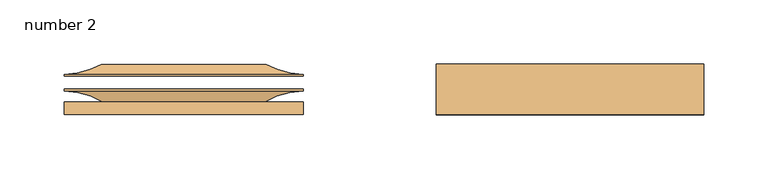
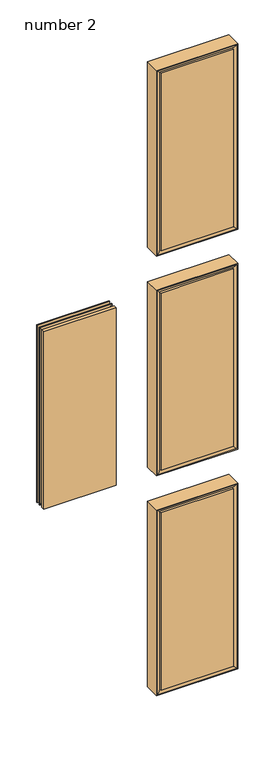
"""IFC4 building model written with IfcOpenShell, lengths in millimetres: door geometry, Door-Interior-Karona-K5660-6_Panel : number 2."""

from ifc_helpers import new_model, si_unit, frame, origin, place, context, project, spatial, polyline, ellipse_curve, source, transform, mapped, element, save
from ifc_brep_helpers import plane_surface, cylinder_surface, revolved_surface, advanced_brep


def number_2_60c607bd(model_context):
    return source(origin(), model_context, "Body", "AdvancedBrep", [
        advanced_brep(
        [(242.8748, -54.4576, 1893.8748), (57.1627, -54.4576, 1893.8748), (57.1627, -54.4576, 1414.4752), (242.8748, -54.4576, 1414.4752), (242.8748, -34.7218, 1893.8748), (57.1627, -34.7218, 1893.8748), (57.1627, -36.0454899, 1893.8748), (242.8748, -36.0454899, 1893.8748), (242.8748, -44.5515929, 1893.8748), (57.1627, -44.5515929, 1893.8748), (57.1627, -34.7218, 1414.4752), (242.8748, -34.7218, 1414.4752), (242.8748, -36.0454899, 1414.4752), (57.1627, -36.0454899, 1414.4752), (57.1627, -44.5515929, 1414.4752), (242.8748, -44.5515929, 1414.4752), (87.1686653, -44.5515929, 1863.8688347), (212.8688347, -44.5515929, 1863.8688347), (87.1686653, -44.5515929, 1444.4811653), (212.8688347, -44.5515929, 1444.4811653)],
        [
            (0, 1),
            (1, 2),
            (2, 3),
            (3, 0),
            (4, 5),
            (5, 6),
            (6, 7),
            (7, 4),
            (0, 8),
            (8, 9),
            (9, 1),
            (10, 11),
            (11, 12),
            (12, 13),
            (13, 10),
            (2, 14),
            (14, 15),
            (15, 3),
            (15, 8),
            (11, 4),
            (7, 12),
            (9, 14),
            (5, 10),
            (13, 6),
            (16, 17),
            (17, 7, ellipse_curve(frame((244.8131685, -100.0605261, 1895.8131685), z_axis=(0.7071067811865475, 0.0, -0.7071067811865475), x_axis=(0.7071067811865476, 0.0, 0.7071067811865474)), 90.5724254, 64.0443762)),
            (6, 16, ellipse_curve(frame((55.2243315, -100.0605261, 1895.8131685), z_axis=(-0.7071067811865475, 0.0, -0.7071067811865475), x_axis=(0.7071067811865476, 0.0, -0.7071067811865474)), 90.5724254, 64.0443762)),
            (18, 16),
            (13, 18, ellipse_curve(frame((55.2243315, -100.0605261, 1412.5368315), z_axis=(0.7071067811865475, 0.0, -0.7071067811865475), x_axis=(0.7071067811865474, 0.0, 0.7071067811865476)), 90.5724254, 64.0443762)),
            (19, 18),
            (12, 19, ellipse_curve(frame((244.8131685, -100.0605261, 1412.5368315), z_axis=(0.7071067811865475, 0.0, 0.7071067811865475), x_axis=(-0.7071067811865476, 0.0, 0.7071067811865474)), 90.5724254, 64.0443762)),
            (17, 19),
        ],
        [
            plane_surface(frame((57.1627, -54.4576, 1893.8748), z_axis=(0.0, -1.0, 0.0), x_axis=(0.0, 0.0, -1.0))),
            plane_surface(frame((57.1627, -34.7218, 1893.8748), z_axis=(0.0, 0.0, 1.0), x_axis=(-1.0, 0.0, 0.0))),
            plane_surface(frame((57.1627, -34.7218, 1414.4752), z_axis=(0.0, 0.0, -1.0), x_axis=(1.0, 0.0, 0.0))),
            plane_surface(frame((242.8748, -54.4576, 1893.8748), z_axis=(1.0, 0.0, 0.0), x_axis=(0.0, 0.0, -1.0))),
            plane_surface(frame((57.1627, -34.7218, 1893.8748), z_axis=(-1.0, 0.0, 0.0), x_axis=(0.0, 0.0, -1.0))),
            plane_surface(frame((242.8748, -34.7218, 1893.8748), z_axis=(0.0, 1.0, 0.0), x_axis=(0.0, 0.0, -1.0))),
            revolved_surface(polyline([(308.8575446888527, -100.0605261, 1831.7687923), (-8.820044688852704, -100.0605261, 1831.7687923)]), (254.0, -100.0605261, 1895.8131685), (1.0, 0.0, 0.0)),
            revolved_surface(polyline([(119.2687077, -100.0605261, 1959.8575446888528), (119.2687077, -100.0605261, 1348.4924553111473)]), (55.2243315, -100.0605261, 1905.0), (0.0, 0.0, 1.0)),
            revolved_surface(polyline([(-8.820044688852683, -100.0605261, 1476.5812077), (308.8575446888527, -100.0605261, 1476.5812077)]), (46.0375, -100.0605261, 1412.5368315), (-1.0, 0.0, 0.0)),
            revolved_surface(polyline([(180.76879229999997, -100.0605261, 1348.4924553111473), (180.76879229999997, -100.0605261, 1959.8575446888526)]), (244.8131685, -100.0605261, 1403.35), (0.0, 0.0, -1.0)),
            plane_surface(frame((254.0, -44.5515929, 1403.35), z_axis=(0.0, 1.0, 0.0), x_axis=(0.0, 0.0, 1.0))),
        ],
        [
            (0, [[1, 2, 3, 4]]),
            (1, [[5, 6, 7, 8]]),
            (1, [[-1, 9, 10, 11]]),
            (2, [[12, 13, 14, 15]]),
            (2, [[-3, 16, 17, 18]]),
            (3, [[-4, -18, 19, -9]]),
            (3, [[20, -8, 21, -13]]),
            (4, [[-2, -11, 22, -16]]),
            (4, [[23, -15, 24, -6]]),
            (5, [[-5, -20, -12, -23]]),
            (6, [[25, 26, -7, 27]]),
            (7, [[28, -27, -24, 29]]),
            (8, [[30, -29, -14, 31]]),
            (9, [[32, -31, -21, -26]]),
            (10, [[-10, -19, -17, -22], [-25, -28, -30, -32]]),
        ],
    ),
        advanced_brep(
        [(242.8748, -24.6126, 1893.8748), (57.1627, -24.6126, 1893.8748), (57.1627, -24.6126, 1414.4752), (242.8748, -24.6126, 1414.4752), (214.0448579, -15.4432, 1443.3051421), (85.9926421, -15.4432, 1443.3051421), (85.9926421, -15.4432, 1865.0448579), (214.0448579, -15.4432, 1865.0448579), (242.8748, -23.2889101, 1893.8748), (57.1627, -23.2889101, 1893.8748), (57.1627, -23.2889101, 1414.4752), (242.8748, -23.2889101, 1414.4752)],
        [
            (0, 1),
            (1, 2),
            (2, 3),
            (3, 0),
            (4, 5),
            (5, 6),
            (6, 7),
            (7, 4),
            (0, 8),
            (8, 9),
            (9, 1),
            (2, 10),
            (10, 11),
            (11, 3),
            (4, 11, ellipse_curve(frame((244.8131685, 40.7261261, 1412.5368315), z_axis=(0.7071067811865475, 0.0, 0.7071067811865475), x_axis=(-0.7071067811865476, 0.0, 0.7071067811865474)), 90.5724254, 64.0443762)),
            (10, 5, ellipse_curve(frame((55.2243315, 40.7261261, 1412.5368315), z_axis=(-0.7071067811865475, 0.0, 0.7071067811865475), x_axis=(-0.7071067811865476, 0.0, -0.7071067811865474)), 90.5724254, 64.0443762)),
            (7, 8, ellipse_curve(frame((244.8131685, 40.7261261, 1895.8131685), z_axis=(-0.7071067811865475, 0.0, 0.7071067811865475), x_axis=(-0.7071067811865474, 0.0, -0.7071067811865476)), 90.5724254, 64.0443762)),
            (8, 11),
            (6, 9, ellipse_curve(frame((55.2243315, 40.7261261, 1895.8131685), z_axis=(-0.7071067811865475, 0.0, -0.7071067811865475), x_axis=(0.7071067811865476, 0.0, -0.7071067811865474)), 90.5724254, 64.0443762)),
            (10, 9),
        ],
        [
            plane_surface(frame((57.1627, -24.6126, 1893.8748), z_axis=(0.0, -1.0, 0.0), x_axis=(0.0, 0.0, -1.0))),
            plane_surface(frame((242.8748, -15.4432, 1893.8748), z_axis=(0.0, 1.0, 0.0), x_axis=(0.0, 0.0, -1.0))),
            plane_surface(frame((57.1627, -34.7218, 1893.8748), z_axis=(0.0, 0.0, 1.0), x_axis=(-1.0, 0.0, 0.0))),
            plane_surface(frame((57.1627, -34.7218, 1414.4752), z_axis=(0.0, 0.0, -1.0), x_axis=(1.0, 0.0, 0.0))),
            revolved_surface(polyline([(-8.820044688852711, 40.7261261, 1476.5812077), (308.8575446888527, 40.7261261, 1476.5812077)]), (46.0375, 40.7261261, 1412.5368315), (-1.0, 0.0, 0.0)),
            revolved_surface(polyline([(180.76879229999997, 40.7261261, 1348.4924553111473), (180.76879229999997, 40.7261261, 1959.8575446888528)]), (244.8131685, 40.7261261, 1403.35), (0.0, 0.0, -1.0)),
            revolved_surface(polyline([(308.85754468885267, 40.7261261, 1831.7687923), (-8.820044688852704, 40.7261261, 1831.7687923)]), (254.0, 40.7261261, 1895.8131685), (1.0, 0.0, 0.0)),
            revolved_surface(polyline([(119.2687077, 40.7261261, 1959.8575446888528), (119.2687077, 40.7261261, 1348.4924553111473)]), (55.2243315, 40.7261261, 1905.0), (0.0, 0.0, 1.0)),
            plane_surface(frame((242.8748, -24.6126, 1893.8748), z_axis=(1.0, 0.0, 0.0), x_axis=(0.0, 0.0, -1.0))),
            plane_surface(frame((57.1627, -15.4432, 1893.8748), z_axis=(-1.0, 0.0, 0.0), x_axis=(0.0, 0.0, -1.0))),
        ],
        [
            (0, [[1, 2, 3, 4]]),
            (1, [[5, 6, 7, 8]]),
            (2, [[-1, 9, 10, 11]]),
            (3, [[-3, 12, 13, 14]]),
            (4, [[15, -13, 16, -5]]),
            (5, [[-15, -8, 17, 18]]),
            (6, [[-17, -7, 19, -10]]),
            (7, [[-19, -6, -16, 20]]),
            (8, [[-4, -14, -18, -9]]),
            (9, [[-2, -11, -20, -12]]),
        ],
    ),
        advanced_brep(
        [(254.0, -15.2908, 1905.0), (242.6746863, -24.6126, 1893.6746863), (57.3628137, -24.6126, 1893.6746863), (46.0375, -15.2908, 1905.0), (57.1627, -46.3324899, 1893.8748), (48.2727, -54.4576, 1902.7648), (48.2727, -54.4576, 1405.5852), (57.1627, -46.3324899, 1414.4752), (242.8748, -46.3324899, 1414.4752), (251.7648, -54.4576, 1405.5852), (251.7648, -54.4576, 1902.7648), (242.8748, -46.3324899, 1893.8748), (46.0375, -54.4576, 1403.35), (46.0375, -15.2908, 1403.35), (254.0, -15.2908, 1403.35), (254.0, -54.4576, 1403.35), (57.1627, -34.7218, 1414.4752), (242.8748, -34.7218, 1414.4752), (47.3075, -24.6126, 1903.73), (47.3075, -34.7218, 1903.73), (47.3075, -34.7218, 1404.62), (47.3075, -24.6126, 1404.62), (252.73, -24.6126, 1404.62), (252.73, -24.6126, 1903.73), (57.3628137, -24.6126, 1414.6753137), (242.6746863, -24.6126, 1414.6753137), (252.73, -34.7218, 1404.62), (254.0, -54.4576, 1905.0), (242.8748, -34.7218, 1893.8748), (252.73, -34.7218, 1903.73), (46.0375, -54.4576, 1905.0), (57.1627, -34.7218, 1893.8748)],
        [
            (0, 1, ellipse_curve(frame((252.9689876, -25.5788135, 1903.9689876), z_axis=(-0.7071067811865475, 0.0, 0.7071067811865475), x_axis=(0.7071067811865476, 0.0, 0.7071067811865474)), 14.6223259, 10.3395458)),
            (1, 2),
            (2, 3, ellipse_curve(frame((47.0685124, -25.5788135, 1903.9689876), z_axis=(0.7071067811865475, 0.0, 0.7071067811865475), x_axis=(0.7071067811865476, 0.0, -0.7071067811865474)), 14.6223259, 10.3395458)),
            (3, 0),
            (4, 5, ellipse_curve(frame((48.2727, -45.531597, 1902.7648), z_axis=(-0.7071067811865475, 0.0, -0.7071067811865475), x_axis=(-0.7071067811865474, 0.0, 0.7071067811865476)), 12.6232745, 8.926003)),
            (5, 6),
            (6, 7, ellipse_curve(frame((48.2727, -45.531597, 1405.5852), z_axis=(-0.7071067811865475, 0.0, 0.7071067811865475), x_axis=(0.7071067811865474, 0.0, 0.7071067811865476)), 12.6232745, 8.926003)),
            (7, 4),
            (8, 9, ellipse_curve(frame((251.7648, -45.531597, 1405.5852), z_axis=(0.7071067811865475, 0.0, 0.7071067811865475), x_axis=(0.7071067811865474, 0.0, -0.7071067811865476)), 12.6232745, 8.926003)),
            (9, 10),
            (10, 11, ellipse_curve(frame((251.7648, -45.531597, 1902.7648), z_axis=(0.7071067811865475, 0.0, -0.7071067811865475), x_axis=(-0.7071067811865474, 0.0, -0.7071067811865476)), 12.6232745, 8.926003)),
            (11, 8),
            (12, 13),
            (13, 14),
            (14, 15),
            (15, 12),
            (16, 7),
            (7, 8),
            (8, 17),
            (17, 16),
            (18, 19),
            (19, 20),
            (20, 21),
            (21, 18),
            (22, 23),
            (23, 18),
            (21, 22),
            (24, 2),
            (1, 25),
            (25, 24),
            (20, 26),
            (26, 22),
            (14, 0),
            (0, 27),
            (27, 15),
            (11, 28),
            (28, 17),
            (26, 29),
            (29, 23),
            (3, 30),
            (30, 27),
            (11, 4),
            (4, 31),
            (31, 28),
            (29, 19),
            (3, 13),
            (12, 30),
            (16, 31),
            (5, 10),
            (9, 6),
            (13, 24, ellipse_curve(frame((47.0685124, -25.5788135, 1404.3810124), z_axis=(0.7071067811865475, 0.0, -0.7071067811865475), x_axis=(-0.7071067811865476, 0.0, -0.7071067811865474)), 14.6223259, 10.3395458)),
            (25, 14, ellipse_curve(frame((252.9689876, -25.5788135, 1404.3810124), z_axis=(-0.7071067811865475, 0.0, -0.7071067811865475), x_axis=(-0.7071067811865476, 0.0, 0.7071067811865474)), 14.6223259, 10.3395458)),
        ],
        [
            cylinder_surface(frame((254.0, -25.5788135, 1903.9689876), z_axis=(1.0, 0.0, 0.0), x_axis=(0.0, 1.0, 0.0)), 10.3395458),
            cylinder_surface(frame((48.2727, -45.531597, 1905.0), z_axis=(0.0, 0.0, 1.0), x_axis=(0.0, 1.0, 0.0)), 8.926003),
            cylinder_surface(frame((251.7648, -45.531597, 1403.35), z_axis=(0.0, 0.0, -1.0), x_axis=(0.0, 1.0, 0.0)), 8.926003),
            plane_surface(frame((46.0375, -15.2908, 1403.35), z_axis=(0.0, 0.0, -1.0), x_axis=(1.0, 0.0, 0.0))),
            plane_surface(frame((57.1627, -46.3324899, 1414.4752), z_axis=(0.0, 0.0, 1.0), x_axis=(1.0, 0.0, 0.0))),
            plane_surface(frame((47.3075, -34.7218, 1903.73), z_axis=(1.0, 0.0, 0.0), x_axis=(0.0, 0.0, -1.0))),
            plane_surface(frame((47.3075, -24.6126, 1903.73), z_axis=(0.0, -1.0, 0.0), x_axis=(0.0, 0.0, -1.0))),
            plane_surface(frame((47.3075, -34.7218, 1404.62), z_axis=(0.0, 0.0, 1.0), x_axis=(1.0, 0.0, 0.0))),
            plane_surface(frame((254.0, -15.2908, 1403.35), z_axis=(1.0, 0.0, 0.0), x_axis=(0.0, 0.0, 1.0))),
            plane_surface(frame((242.8748, -46.3324899, 1414.4752), z_axis=(-1.0, 0.0, 0.0), x_axis=(0.0, 0.0, 1.0))),
            plane_surface(frame((252.73, -34.7218, 1404.62), z_axis=(-1.0, 0.0, 0.0), x_axis=(0.0, 0.0, 1.0))),
            plane_surface(frame((254.0, -15.2908, 1905.0), z_axis=(0.0, 0.0, 1.0), x_axis=(-1.0, 0.0, 0.0))),
            plane_surface(frame((242.8748, -46.3324899, 1893.8748), z_axis=(0.0, 0.0, -1.0), x_axis=(-1.0, 0.0, 0.0))),
            plane_surface(frame((252.73, -34.7218, 1903.73), z_axis=(0.0, 0.0, -1.0), x_axis=(-1.0, 0.0, 0.0))),
            plane_surface(frame((46.0375, -15.2908, 1905.0), z_axis=(-1.0, 0.0, 0.0), x_axis=(0.0, 0.0, -1.0))),
            plane_surface(frame((57.1627, -46.3324899, 1893.8748), z_axis=(1.0, 0.0, 0.0), x_axis=(0.0, 0.0, -1.0))),
            plane_surface(frame((57.1627, -34.7218, 1893.8748), z_axis=(0.0, 1.0, 0.0), x_axis=(0.0, 0.0, -1.0))),
            plane_surface(frame((46.0375, -54.4576, 1905.0), z_axis=(0.0, -1.0, 0.0), x_axis=(0.0, 0.0, -1.0))),
            cylinder_surface(frame((46.0375, -45.531597, 1405.5852), z_axis=(-1.0, 0.0, 0.0), x_axis=(0.0, 1.0, 0.0)), 8.926003),
            cylinder_surface(frame((46.0375, -25.5788135, 1404.3810124), z_axis=(-1.0, 0.0, 0.0), x_axis=(0.0, 1.0, 0.0)), 10.3395458),
            cylinder_surface(frame((252.9689876, -25.5788135, 1403.35), z_axis=(0.0, 0.0, -1.0), x_axis=(0.0, 1.0, 0.0)), 10.3395458),
            cylinder_surface(frame((254.0, -45.531597, 1902.7648), z_axis=(1.0, 0.0, 0.0), x_axis=(0.0, 1.0, 0.0)), 8.926003),
            cylinder_surface(frame((47.0685124, -25.5788135, 1905.0), z_axis=(0.0, 0.0, 1.0), x_axis=(0.0, 1.0, 0.0)), 10.3395458),
        ],
        [
            (0, [[1, 2, 3, 4]]),
            (1, [[5, 6, 7, 8]]),
            (2, [[9, 10, 11, 12]]),
            (3, [[13, 14, 15, 16]]),
            (4, [[17, 18, 19, 20]]),
            (5, [[21, 22, 23, 24]]),
            (6, [[25, 26, -24, 27], [28, -2, 29, 30]]),
            (7, [[-23, 31, 32, -27]]),
            (8, [[-15, 33, 34, 35]]),
            (9, [[-19, -12, 36, 37]]),
            (10, [[-32, 38, 39, -25]]),
            (11, [[-34, -4, 40, 41]]),
            (12, [[-36, 42, 43, 44]]),
            (13, [[-39, 45, -21, -26]]),
            (14, [[-40, 46, -13, 47]]),
            (15, [[-43, -8, -17, 48]]),
            (16, [[-22, -45, -38, -31], [-37, -44, -48, -20]]),
            (17, [[-35, -41, -47, -16], [-6, 49, -10, 50]]),
            (18, [[-7, -50, -9, -18]]),
            (19, [[51, -30, 52, -14]]),
            (20, [[-52, -29, -1, -33]]),
            (21, [[-11, -49, -5, -42]]),
            (22, [[-3, -28, -51, -46]]),
        ],
    ),
        advanced_brep(
        [(242.8748, -54.4576, 1300.1498), (57.1627, -54.4576, 1300.1498), (57.1627, -54.4576, 820.7502), (242.8748, -54.4576, 820.7502), (242.8748, -34.7218, 1300.1498), (57.1627, -34.7218, 1300.1498), (57.1627, -36.0454899, 1300.1498), (242.8748, -36.0454899, 1300.1498), (242.8748, -44.5515929, 1300.1498), (57.1627, -44.5515929, 1300.1498), (57.1627, -34.7218, 820.7502), (242.8748, -34.7218, 820.7502), (242.8748, -36.0454899, 820.7502), (57.1627, -36.0454899, 820.7502), (57.1627, -44.5515929, 820.7502), (242.8748, -44.5515929, 820.7502), (87.1686653, -44.5515929, 1270.1438347), (212.8688347, -44.5515929, 1270.1438347), (87.1686653, -44.5515929, 850.7561653), (212.8688347, -44.5515929, 850.7561653)],
        [
            (0, 1),
            (1, 2),
            (2, 3),
            (3, 0),
            (4, 5),
            (5, 6),
            (6, 7),
            (7, 4),
            (0, 8),
            (8, 9),
            (9, 1),
            (10, 11),
            (11, 12),
            (12, 13),
            (13, 10),
            (2, 14),
            (14, 15),
            (15, 3),
            (15, 8),
            (11, 4),
            (7, 12),
            (9, 14),
            (5, 10),
            (13, 6),
            (16, 17),
            (17, 7, ellipse_curve(frame((244.8131685, -100.0605261, 1302.0881685), z_axis=(0.7071067811865475, 0.0, -0.7071067811865475), x_axis=(0.7071067811865476, 0.0, 0.7071067811865474)), 90.5724254, 64.0443762)),
            (6, 16, ellipse_curve(frame((55.2243315, -100.0605261, 1302.0881685), z_axis=(-0.7071067811865475, 0.0, -0.7071067811865475), x_axis=(0.7071067811865476, 0.0, -0.7071067811865474)), 90.5724254, 64.0443762)),
            (18, 16),
            (13, 18, ellipse_curve(frame((55.2243315, -100.0605261, 818.8118315), z_axis=(0.7071067811865475, 0.0, -0.7071067811865475), x_axis=(0.7071067811865474, 0.0, 0.7071067811865476)), 90.5724254, 64.0443762)),
            (19, 18),
            (12, 19, ellipse_curve(frame((244.8131685, -100.0605261, 818.8118315), z_axis=(0.7071067811865475, 0.0, 0.7071067811865475), x_axis=(-0.7071067811865476, 0.0, 0.7071067811865474)), 90.5724254, 64.0443762)),
            (17, 19),
        ],
        [
            plane_surface(frame((57.1627, -54.4576, 1300.1498), z_axis=(0.0, -1.0, 0.0), x_axis=(0.0, 0.0, -1.0))),
            plane_surface(frame((57.1627, -34.7218, 1300.1498), z_axis=(0.0, 0.0, 1.0), x_axis=(-1.0, 0.0, 0.0))),
            plane_surface(frame((57.1627, -34.7218, 820.7502), z_axis=(0.0, 0.0, -1.0), x_axis=(1.0, 0.0, 0.0))),
            plane_surface(frame((242.8748, -54.4576, 1300.1498), z_axis=(1.0, 0.0, 0.0), x_axis=(0.0, 0.0, -1.0))),
            plane_surface(frame((57.1627, -34.7218, 1300.1498), z_axis=(-1.0, 0.0, 0.0), x_axis=(0.0, 0.0, -1.0))),
            plane_surface(frame((242.8748, -34.7218, 1300.1498), z_axis=(0.0, 1.0, 0.0), x_axis=(0.0, 0.0, -1.0))),
            revolved_surface(polyline([(308.8575446888527, -100.0605261, 1238.0437923), (-8.820044688852704, -100.0605261, 1238.0437923)]), (254.0, -100.0605261, 1302.0881685), (1.0, 0.0, 0.0)),
            revolved_surface(polyline([(119.2687077, -100.0605261, 1366.1325446888527), (119.2687077, -100.0605261, 754.7674553111474)]), (55.2243315, -100.0605261, 1311.275), (0.0, 0.0, 1.0)),
            revolved_surface(polyline([(-8.820044688852683, -100.0605261, 882.8562077), (308.8575446888527, -100.0605261, 882.8562077)]), (46.0375, -100.0605261, 818.8118315), (-1.0, 0.0, 0.0)),
            revolved_surface(polyline([(180.76879229999997, -100.0605261, 754.7674553111474), (180.76879229999997, -100.0605261, 1366.1325446888527)]), (244.8131685, -100.0605261, 809.625), (0.0, 0.0, -1.0)),
            plane_surface(frame((254.0, -44.5515929, 809.625), z_axis=(0.0, 1.0, 0.0), x_axis=(0.0, 0.0, 1.0))),
        ],
        [
            (0, [[1, 2, 3, 4]]),
            (1, [[5, 6, 7, 8]]),
            (1, [[-1, 9, 10, 11]]),
            (2, [[12, 13, 14, 15]]),
            (2, [[-3, 16, 17, 18]]),
            (3, [[-4, -18, 19, -9]]),
            (3, [[20, -8, 21, -13]]),
            (4, [[-2, -11, 22, -16]]),
            (4, [[23, -15, 24, -6]]),
            (5, [[-5, -20, -12, -23]]),
            (6, [[25, 26, -7, 27]]),
            (7, [[28, -27, -24, 29]]),
            (8, [[30, -29, -14, 31]]),
            (9, [[32, -31, -21, -26]]),
            (10, [[-10, -19, -17, -22], [-25, -28, -30, -32]]),
        ],
    ),
        advanced_brep(
        [(242.8748, -24.6126, 1300.1498), (57.1627, -24.6126, 1300.1498), (57.1627, -24.6126, 820.7502), (242.8748, -24.6126, 820.7502), (214.0448579, -15.4432, 849.5801421), (85.9926421, -15.4432, 849.5801421), (85.9926421, -15.4432, 1271.3198579), (214.0448579, -15.4432, 1271.3198579), (242.8748, -23.2889101, 1300.1498), (57.1627, -23.2889101, 1300.1498), (57.1627, -23.2889101, 820.7502), (242.8748, -23.2889101, 820.7502)],
        [
            (0, 1),
            (1, 2),
            (2, 3),
            (3, 0),
            (4, 5),
            (5, 6),
            (6, 7),
            (7, 4),
            (0, 8),
            (8, 9),
            (9, 1),
            (2, 10),
            (10, 11),
            (11, 3),
            (4, 11, ellipse_curve(frame((244.8131685, 40.7261261, 818.8118315), z_axis=(0.7071067811865475, 0.0, 0.7071067811865475), x_axis=(-0.7071067811865476, 0.0, 0.7071067811865474)), 90.5724254, 64.0443762)),
            (10, 5, ellipse_curve(frame((55.2243315, 40.7261261, 818.8118315), z_axis=(-0.7071067811865475, 0.0, 0.7071067811865475), x_axis=(-0.7071067811865476, 0.0, -0.7071067811865474)), 90.5724254, 64.0443762)),
            (7, 8, ellipse_curve(frame((244.8131685, 40.7261261, 1302.0881685), z_axis=(-0.7071067811865475, 0.0, 0.7071067811865475), x_axis=(-0.7071067811865474, 0.0, -0.7071067811865476)), 90.5724254, 64.0443762)),
            (8, 11),
            (6, 9, ellipse_curve(frame((55.2243315, 40.7261261, 1302.0881685), z_axis=(-0.7071067811865475, 0.0, -0.7071067811865475), x_axis=(0.7071067811865476, 0.0, -0.7071067811865474)), 90.5724254, 64.0443762)),
            (10, 9),
        ],
        [
            plane_surface(frame((57.1627, -24.6126, 1300.1498), z_axis=(0.0, -1.0, 0.0), x_axis=(0.0, 0.0, -1.0))),
            plane_surface(frame((242.8748, -15.4432, 1300.1498), z_axis=(0.0, 1.0, 0.0), x_axis=(0.0, 0.0, -1.0))),
            plane_surface(frame((57.1627, -34.7218, 1300.1498), z_axis=(0.0, 0.0, 1.0), x_axis=(-1.0, 0.0, 0.0))),
            plane_surface(frame((57.1627, -34.7218, 820.7502), z_axis=(0.0, 0.0, -1.0), x_axis=(1.0, 0.0, 0.0))),
            revolved_surface(polyline([(-8.820044688852711, 40.7261261, 882.8562077), (308.8575446888527, 40.7261261, 882.8562077)]), (46.0375, 40.7261261, 818.8118315), (-1.0, 0.0, 0.0)),
            revolved_surface(polyline([(180.76879229999997, 40.7261261, 754.7674553111474), (180.76879229999997, 40.7261261, 1366.1325446888527)]), (244.8131685, 40.7261261, 809.625), (0.0, 0.0, -1.0)),
            revolved_surface(polyline([(308.85754468885267, 40.7261261, 1238.0437923), (-8.820044688852704, 40.7261261, 1238.0437923)]), (254.0, 40.7261261, 1302.0881685), (1.0, 0.0, 0.0)),
            revolved_surface(polyline([(119.2687077, 40.7261261, 1366.1325446888527), (119.2687077, 40.7261261, 754.7674553111474)]), (55.2243315, 40.7261261, 1311.275), (0.0, 0.0, 1.0)),
            plane_surface(frame((242.8748, -24.6126, 1300.1498), z_axis=(1.0, 0.0, 0.0), x_axis=(0.0, 0.0, -1.0))),
            plane_surface(frame((57.1627, -15.4432, 1300.1498), z_axis=(-1.0, 0.0, 0.0), x_axis=(0.0, 0.0, -1.0))),
        ],
        [
            (0, [[1, 2, 3, 4]]),
            (1, [[5, 6, 7, 8]]),
            (2, [[-1, 9, 10, 11]]),
            (3, [[-3, 12, 13, 14]]),
            (4, [[15, -13, 16, -5]]),
            (5, [[-15, -8, 17, 18]]),
            (6, [[-17, -7, 19, -10]]),
            (7, [[-19, -6, -16, 20]]),
            (8, [[-4, -14, -18, -9]]),
            (9, [[-2, -11, -20, -12]]),
        ],
    ),
        advanced_brep(
        [(254.0, -15.2908, 1311.275), (242.6746863, -24.6126, 1299.9496863), (57.3628137, -24.6126, 1299.9496863), (46.0375, -15.2908, 1311.275), (57.1627, -46.3324899, 1300.1498), (48.2727, -54.4576, 1309.0398), (48.2727, -54.4576, 811.8602), (57.1627, -46.3324899, 820.7502), (242.8748, -46.3324899, 820.7502), (251.7648, -54.4576, 811.8602), (251.7648, -54.4576, 1309.0398), (242.8748, -46.3324899, 1300.1498), (46.0375, -54.4576, 809.625), (46.0375, -15.2908, 809.625), (254.0, -15.2908, 809.625), (254.0, -54.4576, 809.625), (57.1627, -34.7218, 820.7502), (242.8748, -34.7218, 820.7502), (47.3075, -24.6126, 1310.005), (47.3075, -34.7218, 1310.005), (47.3075, -34.7218, 810.895), (47.3075, -24.6126, 810.895), (252.73, -24.6126, 810.895), (252.73, -24.6126, 1310.005), (57.3628137, -24.6126, 820.9503137), (242.6746863, -24.6126, 820.9503137), (252.73, -34.7218, 810.895), (254.0, -54.4576, 1311.275), (242.8748, -34.7218, 1300.1498), (252.73, -34.7218, 1310.005), (46.0375, -54.4576, 1311.275), (57.1627, -34.7218, 1300.1498)],
        [
            (0, 1, ellipse_curve(frame((252.9689876, -25.5788135, 1310.2439876), z_axis=(-0.7071067811865475, 0.0, 0.7071067811865475), x_axis=(0.7071067811865476, 0.0, 0.7071067811865474)), 14.6223259, 10.3395458)),
            (1, 2),
            (2, 3, ellipse_curve(frame((47.0685124, -25.5788135, 1310.2439876), z_axis=(0.7071067811865475, 0.0, 0.7071067811865475), x_axis=(0.7071067811865476, 0.0, -0.7071067811865474)), 14.6223259, 10.3395458)),
            (3, 0),
            (4, 5, ellipse_curve(frame((48.2727, -45.531597, 1309.0398), z_axis=(-0.7071067811865475, 0.0, -0.7071067811865475), x_axis=(-0.7071067811865474, 0.0, 0.7071067811865476)), 12.6232745, 8.926003)),
            (5, 6),
            (6, 7, ellipse_curve(frame((48.2727, -45.531597, 811.8602), z_axis=(-0.7071067811865475, 0.0, 0.7071067811865475), x_axis=(0.7071067811865474, 0.0, 0.7071067811865476)), 12.6232745, 8.926003)),
            (7, 4),
            (8, 9, ellipse_curve(frame((251.7648, -45.531597, 811.8602), z_axis=(0.7071067811865475, 0.0, 0.7071067811865475), x_axis=(0.7071067811865474, 0.0, -0.7071067811865476)), 12.6232745, 8.926003)),
            (9, 10),
            (10, 11, ellipse_curve(frame((251.7648, -45.531597, 1309.0398), z_axis=(0.7071067811865475, 0.0, -0.7071067811865475), x_axis=(-0.7071067811865474, 0.0, -0.7071067811865476)), 12.6232745, 8.926003)),
            (11, 8),
            (12, 13),
            (13, 14),
            (14, 15),
            (15, 12),
            (16, 7),
            (7, 8),
            (8, 17),
            (17, 16),
            (18, 19),
            (19, 20),
            (20, 21),
            (21, 18),
            (22, 23),
            (23, 18),
            (21, 22),
            (24, 2),
            (1, 25),
            (25, 24),
            (13, 24, ellipse_curve(frame((47.0685124, -25.5788135, 810.6560124), z_axis=(0.7071067811865475, 0.0, -0.7071067811865475), x_axis=(-0.7071067811865476, 0.0, -0.7071067811865474)), 14.6223259, 10.3395458)),
            (25, 14, ellipse_curve(frame((252.9689876, -25.5788135, 810.6560124), z_axis=(-0.7071067811865475, 0.0, -0.7071067811865475), x_axis=(-0.7071067811865476, 0.0, 0.7071067811865474)), 14.6223259, 10.3395458)),
            (20, 26),
            (26, 22),
            (14, 0),
            (0, 27),
            (27, 15),
            (11, 28),
            (28, 17),
            (26, 29),
            (29, 23),
            (3, 30),
            (30, 27),
            (11, 4),
            (4, 31),
            (31, 28),
            (29, 19),
            (3, 13),
            (12, 30),
            (16, 31),
            (5, 10),
            (9, 6),
        ],
        [
            cylinder_surface(frame((254.0, -25.5788135, 1310.2439876), z_axis=(1.0, 0.0, 0.0), x_axis=(0.0, 1.0, 0.0)), 10.3395458),
            cylinder_surface(frame((48.2727, -45.531597, 1311.275), z_axis=(0.0, 0.0, 1.0), x_axis=(0.0, 1.0, 0.0)), 8.926003),
            cylinder_surface(frame((251.7648, -45.531597, 809.625), z_axis=(0.0, 0.0, -1.0), x_axis=(0.0, 1.0, 0.0)), 8.926003),
            plane_surface(frame((46.0375, -15.2908, 809.625), z_axis=(0.0, 0.0, -1.0), x_axis=(1.0, 0.0, 0.0))),
            plane_surface(frame((57.1627, -46.3324899, 820.7502), z_axis=(0.0, 0.0, 1.0), x_axis=(1.0, 0.0, 0.0))),
            plane_surface(frame((47.3075, -34.7218, 1310.005), z_axis=(1.0, 0.0, 0.0), x_axis=(0.0, 0.0, -1.0))),
            plane_surface(frame((47.3075, -24.6126, 1310.005), z_axis=(0.0, -1.0, 0.0), x_axis=(0.0, 0.0, -1.0))),
            cylinder_surface(frame((46.0375, -25.5788135, 810.6560124), z_axis=(-1.0, 0.0, 0.0), x_axis=(0.0, 1.0, 0.0)), 10.3395458),
            plane_surface(frame((47.3075, -34.7218, 810.895), z_axis=(0.0, 0.0, 1.0), x_axis=(1.0, 0.0, 0.0))),
            plane_surface(frame((254.0, -15.2908, 809.625), z_axis=(1.0, 0.0, 0.0), x_axis=(0.0, 0.0, 1.0))),
            plane_surface(frame((242.8748, -46.3324899, 820.7502), z_axis=(-1.0, 0.0, 0.0), x_axis=(0.0, 0.0, 1.0))),
            plane_surface(frame((252.73, -34.7218, 810.895), z_axis=(-1.0, 0.0, 0.0), x_axis=(0.0, 0.0, 1.0))),
            plane_surface(frame((254.0, -15.2908, 1311.275), z_axis=(0.0, 0.0, 1.0), x_axis=(-1.0, 0.0, 0.0))),
            plane_surface(frame((242.8748, -46.3324899, 1300.1498), z_axis=(0.0, 0.0, -1.0), x_axis=(-1.0, 0.0, 0.0))),
            plane_surface(frame((252.73, -34.7218, 1310.005), z_axis=(0.0, 0.0, -1.0), x_axis=(-1.0, 0.0, 0.0))),
            plane_surface(frame((46.0375, -15.2908, 1311.275), z_axis=(-1.0, 0.0, 0.0), x_axis=(0.0, 0.0, -1.0))),
            plane_surface(frame((57.1627, -46.3324899, 1300.1498), z_axis=(1.0, 0.0, 0.0), x_axis=(0.0, 0.0, -1.0))),
            plane_surface(frame((57.1627, -34.7218, 1300.1498), z_axis=(0.0, 1.0, 0.0), x_axis=(0.0, 0.0, -1.0))),
            plane_surface(frame((46.0375, -54.4576, 1311.275), z_axis=(0.0, -1.0, 0.0), x_axis=(0.0, 0.0, -1.0))),
            cylinder_surface(frame((46.0375, -45.531597, 811.8602), z_axis=(-1.0, 0.0, 0.0), x_axis=(0.0, 1.0, 0.0)), 8.926003),
            cylinder_surface(frame((252.9689876, -25.5788135, 809.625), z_axis=(0.0, 0.0, -1.0), x_axis=(0.0, 1.0, 0.0)), 10.3395458),
            cylinder_surface(frame((254.0, -45.531597, 1309.0398), z_axis=(1.0, 0.0, 0.0), x_axis=(0.0, 1.0, 0.0)), 8.926003),
            cylinder_surface(frame((47.0685124, -25.5788135, 1311.275), z_axis=(0.0, 0.0, 1.0), x_axis=(0.0, 1.0, 0.0)), 10.3395458),
        ],
        [
            (0, [[1, 2, 3, 4]]),
            (1, [[5, 6, 7, 8]]),
            (2, [[9, 10, 11, 12]]),
            (3, [[13, 14, 15, 16]]),
            (4, [[17, 18, 19, 20]]),
            (5, [[21, 22, 23, 24]]),
            (6, [[25, 26, -24, 27], [28, -2, 29, 30]]),
            (7, [[31, -30, 32, -14]]),
            (8, [[-23, 33, 34, -27]]),
            (9, [[-15, 35, 36, 37]]),
            (10, [[-19, -12, 38, 39]]),
            (11, [[-34, 40, 41, -25]]),
            (12, [[-36, -4, 42, 43]]),
            (13, [[-38, 44, 45, 46]]),
            (14, [[-41, 47, -21, -26]]),
            (15, [[-42, 48, -13, 49]]),
            (16, [[-45, -8, -17, 50]]),
            (17, [[-22, -47, -40, -33], [-39, -46, -50, -20]]),
            (18, [[-37, -43, -49, -16], [-6, 51, -10, 52]]),
            (19, [[-7, -52, -9, -18]]),
            (20, [[-32, -29, -1, -35]]),
            (21, [[-11, -51, -5, -44]]),
            (22, [[-3, -28, -31, -48]]),
        ],
    ),
        advanced_brep(
        [(242.8748, -54.4576, 706.4248), (57.1627, -54.4576, 706.4248), (57.1627, -54.4576, 227.0252), (242.8748, -54.4576, 227.0252), (242.8748, -34.7218, 706.4248), (57.1627, -34.7218, 706.4248), (57.1627, -36.0454899, 706.4248), (242.8748, -36.0454899, 706.4248), (242.8748, -44.5515929, 706.4248), (57.1627, -44.5515929, 706.4248), (57.1627, -34.7218, 227.0252), (242.8748, -34.7218, 227.0252), (242.8748, -36.0454899, 227.0252), (57.1627, -36.0454899, 227.0252), (57.1627, -44.5515929, 227.0252), (242.8748, -44.5515929, 227.0252), (87.1686653, -44.5515929, 676.4188347), (212.8688347, -44.5515929, 676.4188347), (87.1686653, -44.5515929, 257.0311653), (212.8688347, -44.5515929, 257.0311653)],
        [
            (0, 1),
            (1, 2),
            (2, 3),
            (3, 0),
            (4, 5),
            (5, 6),
            (6, 7),
            (7, 4),
            (0, 8),
            (8, 9),
            (9, 1),
            (10, 11),
            (11, 12),
            (12, 13),
            (13, 10),
            (2, 14),
            (14, 15),
            (15, 3),
            (15, 8),
            (11, 4),
            (7, 12),
            (9, 14),
            (5, 10),
            (13, 6),
            (16, 17),
            (17, 7, ellipse_curve(frame((244.8131685, -100.0605261, 708.3631685), z_axis=(0.7071067811865475, 0.0, -0.7071067811865475), x_axis=(0.7071067811865476, 0.0, 0.7071067811865474)), 90.5724254, 64.0443762)),
            (6, 16, ellipse_curve(frame((55.2243315, -100.0605261, 708.3631685), z_axis=(-0.7071067811865475, 0.0, -0.7071067811865475), x_axis=(0.7071067811865476, 0.0, -0.7071067811865474)), 90.5724254, 64.0443762)),
            (18, 16),
            (13, 18, ellipse_curve(frame((55.2243315, -100.0605261, 225.0868315), z_axis=(0.7071067811865475, 0.0, -0.7071067811865475), x_axis=(0.7071067811865474, 0.0, 0.7071067811865476)), 90.5724254, 64.0443762)),
            (19, 18),
            (12, 19, ellipse_curve(frame((244.8131685, -100.0605261, 225.0868315), z_axis=(0.7071067811865475, 0.0, 0.7071067811865475), x_axis=(-0.7071067811865476, 0.0, 0.7071067811865474)), 90.5724254, 64.0443762)),
            (17, 19),
        ],
        [
            plane_surface(frame((57.1627, -54.4576, 706.4248), z_axis=(0.0, -1.0, 0.0), x_axis=(0.0, 0.0, -1.0))),
            plane_surface(frame((57.1627, -34.7218, 706.4248), z_axis=(0.0, 0.0, 1.0), x_axis=(-1.0, 0.0, 0.0))),
            plane_surface(frame((57.1627, -34.7218, 227.0252), z_axis=(0.0, 0.0, -1.0), x_axis=(1.0, 0.0, 0.0))),
            plane_surface(frame((242.8748, -54.4576, 706.4248), z_axis=(1.0, 0.0, 0.0), x_axis=(0.0, 0.0, -1.0))),
            plane_surface(frame((57.1627, -34.7218, 706.4248), z_axis=(-1.0, 0.0, 0.0), x_axis=(0.0, 0.0, -1.0))),
            plane_surface(frame((242.8748, -34.7218, 706.4248), z_axis=(0.0, 1.0, 0.0), x_axis=(0.0, 0.0, -1.0))),
            revolved_surface(polyline([(308.8575446888527, -100.0605261, 644.3187923), (-8.820044688852704, -100.0605261, 644.3187923)]), (254.0, -100.0605261, 708.3631685), (1.0, 0.0, 0.0)),
            revolved_surface(polyline([(119.2687077, -100.0605261, 772.4075446888527), (119.2687077, -100.0605261, 161.04245531114725)]), (55.2243315, -100.0605261, 717.55), (0.0, 0.0, 1.0)),
            revolved_surface(polyline([(-8.820044688852683, -100.0605261, 289.1312077), (308.8575446888527, -100.0605261, 289.1312077)]), (46.0375, -100.0605261, 225.0868315), (-1.0, 0.0, 0.0)),
            revolved_surface(polyline([(180.76879229999997, -100.0605261, 161.0424553111473), (180.76879229999997, -100.0605261, 772.4075446888527)]), (244.8131685, -100.0605261, 215.9), (0.0, 0.0, -1.0)),
            plane_surface(frame((254.0, -44.5515929, 215.9), z_axis=(0.0, 1.0, 0.0), x_axis=(0.0, 0.0, 1.0))),
        ],
        [
            (0, [[1, 2, 3, 4]]),
            (1, [[5, 6, 7, 8]]),
            (1, [[-1, 9, 10, 11]]),
            (2, [[12, 13, 14, 15]]),
            (2, [[-3, 16, 17, 18]]),
            (3, [[-4, -18, 19, -9]]),
            (3, [[20, -8, 21, -13]]),
            (4, [[-2, -11, 22, -16]]),
            (4, [[23, -15, 24, -6]]),
            (5, [[-5, -20, -12, -23]]),
            (6, [[25, 26, -7, 27]]),
            (7, [[28, -27, -24, 29]]),
            (8, [[30, -29, -14, 31]]),
            (9, [[32, -31, -21, -26]]),
            (10, [[-10, -19, -17, -22], [-25, -28, -30, -32]]),
        ],
    ),
        advanced_brep(
        [(242.8748, -24.6126, 706.4248), (57.1627, -24.6126, 706.4248), (57.1627, -24.6126, 227.0252), (242.8748, -24.6126, 227.0252), (214.0448579, -15.4432, 255.8551421), (85.9926421, -15.4432, 255.8551421), (85.9926421, -15.4432, 677.5948579), (214.0448579, -15.4432, 677.5948579), (242.8748, -23.2889101, 706.4248), (57.1627, -23.2889101, 706.4248), (57.1627, -23.2889101, 227.0252), (242.8748, -23.2889101, 227.0252)],
        [
            (0, 1),
            (1, 2),
            (2, 3),
            (3, 0),
            (4, 5),
            (5, 6),
            (6, 7),
            (7, 4),
            (0, 8),
            (8, 9),
            (9, 1),
            (2, 10),
            (10, 11),
            (11, 3),
            (4, 11, ellipse_curve(frame((244.8131685, 40.7261261, 225.0868315), z_axis=(0.7071067811865475, 0.0, 0.7071067811865475), x_axis=(-0.7071067811865476, 0.0, 0.7071067811865474)), 90.5724254, 64.0443762)),
            (10, 5, ellipse_curve(frame((55.2243315, 40.7261261, 225.0868315), z_axis=(-0.7071067811865475, 0.0, 0.7071067811865475), x_axis=(-0.7071067811865476, 0.0, -0.7071067811865474)), 90.5724254, 64.0443762)),
            (7, 8, ellipse_curve(frame((244.8131685, 40.7261261, 708.3631685), z_axis=(-0.7071067811865475, 0.0, 0.7071067811865475), x_axis=(-0.7071067811865474, 0.0, -0.7071067811865476)), 90.5724254, 64.0443762)),
            (8, 11),
            (6, 9, ellipse_curve(frame((55.2243315, 40.7261261, 708.3631685), z_axis=(-0.7071067811865475, 0.0, -0.7071067811865475), x_axis=(0.7071067811865476, 0.0, -0.7071067811865474)), 90.5724254, 64.0443762)),
            (10, 9),
        ],
        [
            plane_surface(frame((57.1627, -24.6126, 706.4248), z_axis=(0.0, -1.0, 0.0), x_axis=(0.0, 0.0, -1.0))),
            plane_surface(frame((242.8748, -15.4432, 706.4248), z_axis=(0.0, 1.0, 0.0), x_axis=(0.0, 0.0, -1.0))),
            plane_surface(frame((57.1627, -34.7218, 706.4248), z_axis=(0.0, 0.0, 1.0), x_axis=(-1.0, 0.0, 0.0))),
            plane_surface(frame((57.1627, -34.7218, 227.0252), z_axis=(0.0, 0.0, -1.0), x_axis=(1.0, 0.0, 0.0))),
            revolved_surface(polyline([(-8.820044688852711, 40.7261261, 289.1312077), (308.8575446888527, 40.7261261, 289.1312077)]), (46.0375, 40.7261261, 225.0868315), (-1.0, 0.0, 0.0)),
            revolved_surface(polyline([(180.76879229999997, 40.7261261, 161.0424553111473), (180.76879229999997, 40.7261261, 772.4075446888527)]), (244.8131685, 40.7261261, 215.9), (0.0, 0.0, -1.0)),
            revolved_surface(polyline([(308.85754468885267, 40.7261261, 644.3187923), (-8.820044688852704, 40.7261261, 644.3187923)]), (254.0, 40.7261261, 708.3631685), (1.0, 0.0, 0.0)),
            revolved_surface(polyline([(119.2687077, 40.7261261, 772.4075446888527), (119.2687077, 40.7261261, 161.04245531114736)]), (55.2243315, 40.7261261, 717.55), (0.0, 0.0, 1.0)),
            plane_surface(frame((242.8748, -24.6126, 706.4248), z_axis=(1.0, 0.0, 0.0), x_axis=(0.0, 0.0, -1.0))),
            plane_surface(frame((57.1627, -15.4432, 706.4248), z_axis=(-1.0, 0.0, 0.0), x_axis=(0.0, 0.0, -1.0))),
        ],
        [
            (0, [[1, 2, 3, 4]]),
            (1, [[5, 6, 7, 8]]),
            (2, [[-1, 9, 10, 11]]),
            (3, [[-3, 12, 13, 14]]),
            (4, [[15, -13, 16, -5]]),
            (5, [[-15, -8, 17, 18]]),
            (6, [[-17, -7, 19, -10]]),
            (7, [[-19, -6, -16, 20]]),
            (8, [[-4, -14, -18, -9]]),
            (9, [[-2, -11, -20, -12]]),
        ],
    ),
        advanced_brep(
        [(254.0, -15.2908, 717.55), (242.6746863, -24.6126, 706.2246863), (57.3628137, -24.6126, 706.2246863), (46.0375, -15.2908, 717.55), (57.1627, -46.3324899, 706.4248), (48.2727, -54.4576, 715.3148), (48.2727, -54.4576, 218.1352), (57.1627, -46.3324899, 227.0252), (242.8748, -46.3324899, 227.0252), (251.7648, -54.4576, 218.1352), (251.7648, -54.4576, 715.3148), (242.8748, -46.3324899, 706.4248), (46.0375, -54.4576, 215.9), (46.0375, -15.2908, 215.9), (254.0, -15.2908, 215.9), (254.0, -54.4576, 215.9), (57.1627, -34.7218, 227.0252), (242.8748, -34.7218, 227.0252), (47.3075, -24.6126, 716.28), (47.3075, -34.7218, 716.28), (47.3075, -34.7218, 217.17), (47.3075, -24.6126, 217.17), (252.73, -24.6126, 217.17), (252.73, -24.6126, 716.28), (57.3628137, -24.6126, 227.2253137), (242.6746863, -24.6126, 227.2253137), (252.73, -34.7218, 217.17), (254.0, -54.4576, 717.55), (242.8748, -34.7218, 706.4248), (252.73, -34.7218, 716.28), (46.0375, -54.4576, 717.55), (57.1627, -34.7218, 706.4248)],
        [
            (0, 1, ellipse_curve(frame((252.9689876, -25.5788135, 716.5189876), z_axis=(-0.7071067811865475, 0.0, 0.7071067811865475), x_axis=(0.7071067811865476, 0.0, 0.7071067811865474)), 14.6223259, 10.3395458)),
            (1, 2),
            (2, 3, ellipse_curve(frame((47.0685124, -25.5788135, 716.5189876), z_axis=(0.7071067811865475, 0.0, 0.7071067811865475), x_axis=(0.7071067811865476, 0.0, -0.7071067811865474)), 14.6223259, 10.3395458)),
            (3, 0),
            (4, 5, ellipse_curve(frame((48.2727, -45.531597, 715.3148), z_axis=(-0.7071067811865475, 0.0, -0.7071067811865475), x_axis=(-0.7071067811865474, 0.0, 0.7071067811865476)), 12.6232745, 8.926003)),
            (5, 6),
            (6, 7, ellipse_curve(frame((48.2727, -45.531597, 218.1352), z_axis=(-0.7071067811865475, 0.0, 0.7071067811865475), x_axis=(0.7071067811865474, 0.0, 0.7071067811865476)), 12.6232745, 8.926003)),
            (7, 4),
            (8, 9, ellipse_curve(frame((251.7648, -45.531597, 218.1352), z_axis=(0.7071067811865475, 0.0, 0.7071067811865475), x_axis=(0.7071067811865474, 0.0, -0.7071067811865476)), 12.6232745, 8.926003)),
            (9, 10),
            (10, 11, ellipse_curve(frame((251.7648, -45.531597, 715.3148), z_axis=(0.7071067811865475, 0.0, -0.7071067811865475), x_axis=(-0.7071067811865474, 0.0, -0.7071067811865476)), 12.6232745, 8.926003)),
            (11, 8),
            (12, 13),
            (13, 14),
            (14, 15),
            (15, 12),
            (16, 7),
            (7, 8),
            (8, 17),
            (17, 16),
            (18, 19),
            (19, 20),
            (20, 21),
            (21, 18),
            (22, 23),
            (23, 18),
            (21, 22),
            (24, 2),
            (1, 25),
            (25, 24),
            (13, 24, ellipse_curve(frame((47.0685124, -25.5788135, 216.9310124), z_axis=(0.7071067811865475, 0.0, -0.7071067811865475), x_axis=(-0.7071067811865476, 0.0, -0.7071067811865474)), 14.6223259, 10.3395458)),
            (25, 14, ellipse_curve(frame((252.9689876, -25.5788135, 216.9310124), z_axis=(-0.7071067811865475, 0.0, -0.7071067811865475), x_axis=(-0.7071067811865476, 0.0, 0.7071067811865474)), 14.6223259, 10.3395458)),
            (20, 26),
            (26, 22),
            (14, 0),
            (0, 27),
            (27, 15),
            (11, 28),
            (28, 17),
            (26, 29),
            (29, 23),
            (3, 30),
            (30, 27),
            (11, 4),
            (4, 31),
            (31, 28),
            (29, 19),
            (3, 13),
            (12, 30),
            (16, 31),
            (5, 10),
            (9, 6),
        ],
        [
            cylinder_surface(frame((254.0, -25.5788135, 716.5189876), z_axis=(1.0, 0.0, 0.0), x_axis=(0.0, 1.0, 0.0)), 10.3395458),
            cylinder_surface(frame((48.2727, -45.531597, 717.55), z_axis=(0.0, 0.0, 1.0), x_axis=(0.0, 1.0, 0.0)), 8.926003),
            cylinder_surface(frame((251.7648, -45.531597, 215.9), z_axis=(0.0, 0.0, -1.0), x_axis=(0.0, 1.0, 0.0)), 8.926003),
            plane_surface(frame((46.0375, -15.2908, 215.9), z_axis=(0.0, 0.0, -1.0), x_axis=(1.0, 0.0, 0.0))),
            plane_surface(frame((57.1627, -46.3324899, 227.0252), z_axis=(0.0, 0.0, 1.0), x_axis=(1.0, 0.0, 0.0))),
            plane_surface(frame((47.3075, -34.7218, 716.28), z_axis=(1.0, 0.0, 0.0), x_axis=(0.0, 0.0, -1.0))),
            plane_surface(frame((47.3075, -24.6126, 716.28), z_axis=(0.0, -1.0, 0.0), x_axis=(0.0, 0.0, -1.0))),
            cylinder_surface(frame((46.0375, -25.5788135, 216.9310124), z_axis=(-1.0, 0.0, 0.0), x_axis=(0.0, 1.0, 0.0)), 10.3395458),
            plane_surface(frame((47.3075, -34.7218, 217.17), z_axis=(0.0, 0.0, 1.0), x_axis=(1.0, 0.0, 0.0))),
            plane_surface(frame((254.0, -15.2908, 215.9), z_axis=(1.0, 0.0, 0.0), x_axis=(0.0, 0.0, 1.0))),
            plane_surface(frame((242.8748, -46.3324899, 227.0252), z_axis=(-1.0, 0.0, 0.0), x_axis=(0.0, 0.0, 1.0))),
            plane_surface(frame((252.73, -34.7218, 217.17), z_axis=(-1.0, 0.0, 0.0), x_axis=(0.0, 0.0, 1.0))),
            plane_surface(frame((254.0, -15.2908, 717.55), z_axis=(0.0, 0.0, 1.0), x_axis=(-1.0, 0.0, 0.0))),
            plane_surface(frame((242.8748, -46.3324899, 706.4248), z_axis=(0.0, 0.0, -1.0), x_axis=(-1.0, 0.0, 0.0))),
            plane_surface(frame((252.73, -34.7218, 716.28), z_axis=(0.0, 0.0, -1.0), x_axis=(-1.0, 0.0, 0.0))),
            plane_surface(frame((46.0375, -15.2908, 717.55), z_axis=(-1.0, 0.0, 0.0), x_axis=(0.0, 0.0, -1.0))),
            plane_surface(frame((57.1627, -46.3324899, 706.4248), z_axis=(1.0, 0.0, 0.0), x_axis=(0.0, 0.0, -1.0))),
            plane_surface(frame((57.1627, -34.7218, 706.4248), z_axis=(0.0, 1.0, 0.0), x_axis=(0.0, 0.0, -1.0))),
            plane_surface(frame((46.0375, -54.4576, 717.55), z_axis=(0.0, -1.0, 0.0), x_axis=(0.0, 0.0, -1.0))),
            cylinder_surface(frame((46.0375, -45.531597, 218.1352), z_axis=(-1.0, 0.0, 0.0), x_axis=(0.0, 1.0, 0.0)), 8.926003),
            cylinder_surface(frame((252.9689876, -25.5788135, 215.9), z_axis=(0.0, 0.0, -1.0), x_axis=(0.0, 1.0, 0.0)), 10.3395458),
            cylinder_surface(frame((254.0, -45.531597, 715.3148), z_axis=(1.0, 0.0, 0.0), x_axis=(0.0, 1.0, 0.0)), 8.926003),
            cylinder_surface(frame((47.0685124, -25.5788135, 717.55), z_axis=(0.0, 0.0, 1.0), x_axis=(0.0, 1.0, 0.0)), 10.3395458),
        ],
        [
            (0, [[1, 2, 3, 4]]),
            (1, [[5, 6, 7, 8]]),
            (2, [[9, 10, 11, 12]]),
            (3, [[13, 14, 15, 16]]),
            (4, [[17, 18, 19, 20]]),
            (5, [[21, 22, 23, 24]]),
            (6, [[25, 26, -24, 27], [28, -2, 29, 30]]),
            (7, [[31, -30, 32, -14]]),
            (8, [[-23, 33, 34, -27]]),
            (9, [[-15, 35, 36, 37]]),
            (10, [[-19, -12, 38, 39]]),
            (11, [[-34, 40, 41, -25]]),
            (12, [[-36, -4, 42, 43]]),
            (13, [[-38, 44, 45, 46]]),
            (14, [[-41, 47, -21, -26]]),
            (15, [[-42, 48, -13, 49]]),
            (16, [[-45, -8, -17, 50]]),
            (17, [[-22, -47, -40, -33], [-39, -46, -50, -20]]),
            (18, [[-37, -43, -49, -16], [-6, 51, -10, 52]]),
            (19, [[-7, -52, -9, -18]]),
            (20, [[-32, -29, -1, -35]]),
            (21, [[-11, -51, -5, -44]]),
            (22, [[-3, -28, -31, -48]]),
        ],
    ),
        advanced_brep(
        [(-242.8748, -54.4576, 1300.1498), (-242.8748, -54.4576, 820.7502), (-57.1627, -54.4576, 820.7502), (-57.1627, -54.4576, 1300.1498), (-242.8748, -34.7218, 1300.1498), (-242.8748, -36.0454899, 1300.1498), (-57.1627, -36.0454899, 1300.1498), (-57.1627, -34.7218, 1300.1498), (-57.1627, -44.5515929, 1300.1498), (-242.8748, -44.5515929, 1300.1498), (-57.1627, -34.7218, 820.7502), (-57.1627, -36.0454899, 820.7502), (-242.8748, -36.0454899, 820.7502), (-242.8748, -34.7218, 820.7502), (-242.8748, -44.5515929, 820.7502), (-57.1627, -44.5515929, 820.7502), (-87.1686653, -44.5515929, 1270.1438347), (-212.8688347, -44.5515929, 1270.1438347), (-87.1686653, -44.5515929, 850.7561653), (-212.8688347, -44.5515929, 850.7561653)],
        [
            (0, 1),
            (1, 2),
            (2, 3),
            (3, 0),
            (4, 5),
            (5, 6),
            (6, 7),
            (7, 4),
            (3, 8),
            (8, 9),
            (9, 0),
            (10, 11),
            (11, 12),
            (12, 13),
            (13, 10),
            (1, 14),
            (14, 15),
            (15, 2),
            (9, 14),
            (12, 5),
            (4, 13),
            (6, 11),
            (10, 7),
            (15, 8),
            (16, 6, ellipse_curve(frame((-55.2243315, -100.0605261, 1302.0881685), z_axis=(0.7071067811865475, 0.0, -0.7071067811865475), x_axis=(-0.7071067811865476, 0.0, -0.7071067811865474)), 90.5724254, 64.0443762)),
            (5, 17, ellipse_curve(frame((-244.8131685, -100.0605261, 1302.0881685), z_axis=(-0.7071067811865475, 0.0, -0.7071067811865475), x_axis=(-0.7071067811865476, 0.0, 0.7071067811865474)), 90.5724254, 64.0443762)),
            (17, 16),
            (18, 11, ellipse_curve(frame((-55.2243315, -100.0605261, 818.8118315), z_axis=(-0.7071067811865475, 0.0, -0.7071067811865475), x_axis=(-0.7071067811865474, 0.0, 0.7071067811865476)), 90.5724254, 64.0443762)),
            (16, 18),
            (19, 12, ellipse_curve(frame((-244.8131685, -100.0605261, 818.8118315), z_axis=(-0.7071067811865475, 0.0, 0.7071067811865475), x_axis=(0.7071067811865476, 0.0, 0.7071067811865474)), 90.5724254, 64.0443762)),
            (18, 19),
            (19, 17),
        ],
        [
            plane_surface(frame((-57.1627, -54.4576, 1300.1498), z_axis=(0.0, -1.0, 0.0), x_axis=(0.0, 0.0, -1.0))),
            plane_surface(frame((-57.1627, -34.7218, 1300.1498), z_axis=(0.0, 0.0, 1.0), x_axis=(1.0, 0.0, 0.0))),
            plane_surface(frame((-57.1627, -34.7218, 820.7502), z_axis=(0.0, 0.0, -1.0), x_axis=(-1.0, 0.0, 0.0))),
            plane_surface(frame((-242.8748, -54.4576, 1300.1498), z_axis=(-1.0, 0.0, 0.0), x_axis=(0.0, 0.0, -1.0))),
            plane_surface(frame((-57.1627, -34.7218, 1300.1498), z_axis=(1.0, 0.0, 0.0), x_axis=(0.0, 0.0, -1.0))),
            plane_surface(frame((-242.8748, -34.7218, 1300.1498), z_axis=(0.0, 1.0, 0.0), x_axis=(0.0, 0.0, -1.0))),
            revolved_surface(polyline([(-308.8575446888527, -100.0605261, 1238.0437923), (8.820044688852704, -100.0605261, 1238.0437923)]), (-254.0, -100.0605261, 1302.0881685), (-1.0, 0.0, 0.0)),
            revolved_surface(polyline([(-119.2687077, -100.0605261, 1366.1325446888527), (-119.2687077, -100.0605261, 754.7674553111474)]), (-55.2243315, -100.0605261, 1311.275), (0.0, 0.0, 1.0)),
            revolved_surface(polyline([(8.820044688852683, -100.0605261, 882.8562077), (-308.8575446888527, -100.0605261, 882.8562077)]), (-46.0375, -100.0605261, 818.8118315), (1.0, 0.0, 0.0)),
            revolved_surface(polyline([(-180.76879229999997, -100.0605261, 754.7674553111474), (-180.76879229999997, -100.0605261, 1366.1325446888527)]), (-244.8131685, -100.0605261, 809.625), (0.0, 0.0, -1.0)),
            plane_surface(frame((-254.0, -44.5515929, 809.625), z_axis=(0.0, 1.0, 0.0), x_axis=(0.0, 0.0, 1.0))),
        ],
        [
            (0, [[1, 2, 3, 4]]),
            (1, [[5, 6, 7, 8]]),
            (1, [[9, 10, 11, -4]]),
            (2, [[12, 13, 14, 15]]),
            (2, [[16, 17, 18, -2]]),
            (3, [[-11, 19, -16, -1]]),
            (3, [[-14, 20, -5, 21]]),
            (4, [[-7, 22, -12, 23]]),
            (4, [[-18, 24, -9, -3]]),
            (5, [[-23, -15, -21, -8]]),
            (6, [[25, -6, 26, 27]]),
            (7, [[28, -22, -25, 29]]),
            (8, [[30, -13, -28, 31]]),
            (9, [[-26, -20, -30, 32]]),
            (10, [[-24, -17, -19, -10], [-32, -31, -29, -27]]),
        ],
    ),
        advanced_brep(
        [(-242.8748, -24.6126, 1300.1498), (-242.8748, -24.6126, 820.7502), (-57.1627, -24.6126, 820.7502), (-57.1627, -24.6126, 1300.1498), (-214.0448579, -15.4432, 849.5801421), (-214.0448579, -15.4432, 1271.3198579), (-85.9926421, -15.4432, 1271.3198579), (-85.9926421, -15.4432, 849.5801421), (-57.1627, -23.2889101, 1300.1498), (-242.8748, -23.2889101, 1300.1498), (-242.8748, -23.2889101, 820.7502), (-57.1627, -23.2889101, 820.7502)],
        [
            (0, 1),
            (1, 2),
            (2, 3),
            (3, 0),
            (4, 5),
            (5, 6),
            (6, 7),
            (7, 4),
            (3, 8),
            (8, 9),
            (9, 0),
            (1, 10),
            (10, 11),
            (11, 2),
            (7, 11, ellipse_curve(frame((-55.2243315, 40.7261261, 818.8118315), z_axis=(0.7071067811865475, 0.0, 0.7071067811865475), x_axis=(0.7071067811865476, 0.0, -0.7071067811865474)), 90.5724254, 64.0443762)),
            (10, 4, ellipse_curve(frame((-244.8131685, 40.7261261, 818.8118315), z_axis=(-0.7071067811865475, 0.0, 0.7071067811865475), x_axis=(0.7071067811865476, 0.0, 0.7071067811865474)), 90.5724254, 64.0443762)),
            (10, 9),
            (9, 5, ellipse_curve(frame((-244.8131685, 40.7261261, 1302.0881685), z_axis=(0.7071067811865475, 0.0, 0.7071067811865475), x_axis=(0.7071067811865474, 0.0, -0.7071067811865476)), 90.5724254, 64.0443762)),
            (8, 6, ellipse_curve(frame((-55.2243315, 40.7261261, 1302.0881685), z_axis=(0.7071067811865475, 0.0, -0.7071067811865475), x_axis=(-0.7071067811865476, 0.0, -0.7071067811865474)), 90.5724254, 64.0443762)),
            (8, 11),
        ],
        [
            plane_surface(frame((-57.1627, -24.6126, 1300.1498), z_axis=(0.0, -1.0, 0.0), x_axis=(0.0, 0.0, -1.0))),
            plane_surface(frame((-242.8748, -15.4432, 1300.1498), z_axis=(0.0, 1.0, 0.0), x_axis=(0.0, 0.0, -1.0))),
            plane_surface(frame((-57.1627, -34.7218, 1300.1498), z_axis=(0.0, 0.0, 1.0), x_axis=(1.0, 0.0, 0.0))),
            plane_surface(frame((-57.1627, -34.7218, 820.7502), z_axis=(0.0, 0.0, -1.0), x_axis=(-1.0, 0.0, 0.0))),
            revolved_surface(polyline([(8.820044688852711, 40.7261261, 882.8562077), (-308.8575446888527, 40.7261261, 882.8562077)]), (-46.0375, 40.7261261, 818.8118315), (1.0, 0.0, 0.0)),
            revolved_surface(polyline([(-180.76879229999997, 40.7261261, 754.7674553111474), (-180.76879229999997, 40.7261261, 1366.1325446888527)]), (-244.8131685, 40.7261261, 809.625), (0.0, 0.0, -1.0)),
            revolved_surface(polyline([(-308.85754468885267, 40.7261261, 1238.0437923), (8.820044688852704, 40.7261261, 1238.0437923)]), (-254.0, 40.7261261, 1302.0881685), (-1.0, 0.0, 0.0)),
            revolved_surface(polyline([(-119.2687077, 40.7261261, 1366.1325446888527), (-119.2687077, 40.7261261, 754.7674553111474)]), (-55.2243315, 40.7261261, 1311.275), (0.0, 0.0, 1.0)),
            plane_surface(frame((-242.8748, -24.6126, 1300.1498), z_axis=(-1.0, 0.0, 0.0), x_axis=(0.0, 0.0, -1.0))),
            plane_surface(frame((-57.1627, -15.4432, 1300.1498), z_axis=(1.0, 0.0, 0.0), x_axis=(0.0, 0.0, -1.0))),
        ],
        [
            (0, [[1, 2, 3, 4]]),
            (1, [[5, 6, 7, 8]]),
            (2, [[9, 10, 11, -4]]),
            (3, [[12, 13, 14, -2]]),
            (4, [[-8, 15, -13, 16]]),
            (5, [[17, 18, -5, -16]]),
            (6, [[-10, 19, -6, -18]]),
            (7, [[20, -15, -7, -19]]),
            (8, [[-11, -17, -12, -1]]),
            (9, [[-14, -20, -9, -3]]),
        ],
    ),
    ])


if __name__ == "__main__":
    model = new_model("IFC4")
    model_context = context("Model", 3, world=origin())
    ifc_project = project(units=[si_unit("LENGTHUNIT", "METRE", prefix="MILLI")], contexts=[model_context])
    site = spatial("IfcSite", under=ifc_project)
    building = spatial("IfcBuilding", under=site)
    placement = place(None, origin())
    number_2_shape = number_2_60c607bd(model_context)
    element("IfcDoor", 1, ObjectType="Door-Interior-Karona-K5660-6_Panel : number 2", at=placement, inside=building, context=model_context, shape_type="MappedRepresentation", body=[
        mapped(number_2_shape, transform((0.0, 0.0, 0.0), x_axis=(1.0, 0.0, 0.0), y_axis=(0.0, 1.0, 0.0), z_axis=(0.0, 0.0, 1.0))),
    ])
    save(model, "model.ifc")

# Revit data of these elements
# Type "Door-Interior-Karona-K5660-6_Panel : number 2"
#   Type Mark = "82"
#   Youtube clip = ""
#   Warranty URL = "http://www.karonadoor.com/pdf/literature/Warranty_.pdf"
#   Warranty = "Limited lifetime warranty on all interior doors."
#   Uniformat II Description = ""
#   Uniformat II Code = ""
#   Uniclass 2015 Name = "Doorsets"
#   Uniclass 2015 Code = "Pr_30_59_24"
#   Uniclass 2.0 Description = "Doorsets"
#   Uniclass 2.0 Code = "PR-59-23"
#   Uniclass 1.4 Description = "Doors"
#   Uniclass 1.4 Code = "JL20"
#   URL = "http://www.karonadoor.com/"
#   UNSPSC Code = "30171511"
#   Technical description = "http://www.karonadoor.com/pdf/Architectural.Guide.pdf"
#   Support Email = "mailto:bimsupport@jeldwen.com"
#   Region South America = "None"
#   Region Oceania = "None"
#   Region North America = "CA, US"
#   Region Middle East = "None"
#   Region Europe = "None"
#   Region Asia = "None"
#   Region Antarctica = "None"
#   Region Africa = "None"
#   QR code = "http://bimobject.com/karona/product/K5660"
#   Product url = "http://www.karonadoor.com/commercial_products.php?category_id=1&style_id=1&image_id=21"
#   Product group = "Panel Doors"
#   Product family = "Commercial Products"
#   Product data url = "https://bimobject.com/karona/product/K5660"
#   Product certification = ""
#   Product SKU = "K5660"
#   Product Guid = "0ef6a8f4-4242-4391-b579-45df545b9ddd"
#   Operation = "Swing"
#   OmniClass Description = "Wood Doors"
#   OmniClass Code = "23-17 11 15"
#   NBS Reference Description = "Doorsets"
#   NBS Reference Code = "59-23"
#   Model = "K5660"
#   Material secondary = ""
#   Material main = "Wood"
#   Masterformat 2014 Description = "Stile and Rail Wood Doors"
#   Masterformat 2014 Code = "08 14 33"
#   Manufacturer name = "Karona"
#   Manufacturer country = "United States"
#   Manufacturer = "Karona Door, Inc."
#   Keynote = "08 14 33"
#   Installation instructions = ""
#   IFC Classification = "Door"
#   Green Product Information = "Available in Certified Wood, No-added Urea, & Recycled"
#   Fire Rating Data = "http://www.karonadoor.com/pdf/literature/Fire_Door_Options.pdf"
#   Fire Rating = "Available in 20, 45, 60, & 90 minute ratings."
#   EAN code = ""
#   Design country = "United States"
#   Description = "Commercial 6-Panel Stile and Rail Wood Door"
#   Date of publishing = ""
#   COBIe Type Category = ""
#   Brand url = "http://www.karonadoor.com/"
#   BIMobject main category code = "doors"
#   BIMobject main category = "Doors"
#   BIMobject category code = "doors-swing"
#   BIMobject category = "Swing"
#   Analytic Construction = "Solid core wood"
#   Sticking Profile Note = "Select only one sticking profile."
#   Sizing Statement = "Custom sizes are available."
#   Panel Style Note = "Select only one panel style."
#   Glass Options Note = "19 styles of glass are available."
#   Fire Door Note = "Available in 20, 45, 60, & 90 minute ratings."
#   Trim Width = 0' - 3 21/32"
#   Trim Reveal = 0' - 0 1/4"
#   Trim Offset = 0' - 3"
#   Top Rail Height = 0' - 5"
#   Thermal Resistance (R) = 0.382863 (m²·K)/W
#   Stile Width = 0' - 5"
#   Sticking Offset = 0' - 0 7/16"
#   Raised Panel Offset = 0' - 1 5/8"
#   Panel Height = 1' - 7 3/4"
#   Mullion Width = 0' - 3 5/8"
#   Mid Rail Height = 4' - 7 1/4"
#   Lock Rail Width = 0' - 3 5/8"
#   Lock Rail Height = 2' - 7 7/8"
#   Jamb to Door Gap = 0' - 0 3/64"
#   Hinge Length = 0' - 2 1/4"
